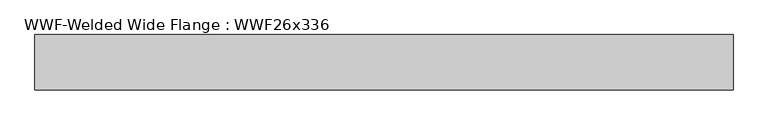
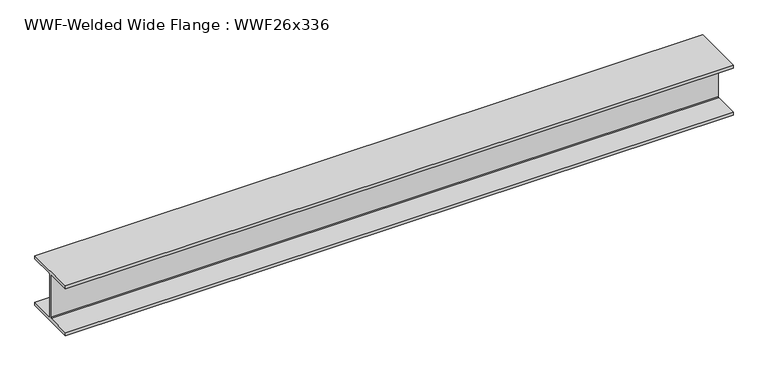
"""IFC4 building model written with IfcOpenShell, lengths in millimetres: beam geometry, WWF-Welded Wide Flange : WWF26x336."""

from ifc_helpers import new_model, si_unit, frame, origin, place, context, project, spatial, polyline, outline, extrude, source, transform, mapped, element, save


def wwf_welded_wide_flange_wwf26x336_e7b07e13(model_context):
    return source(origin(), model_context, "Body", "SweptSolid", [
        extrude(outline(polyline([(324.993, -284.988), (324.993, -324.993), (-324.993, -324.993), (-324.993, -284.988), (-20.6375, -284.988), (-9.9949, -274.3454), (-9.9949, 274.3454), (-20.6375, 284.988), (-324.993, 284.988), (-324.993, 324.993), (324.993, 324.993), (324.993, 284.988), (20.6375, 284.988), (9.9949, 274.3454), (9.9949, -274.3454), (20.6375, -284.988), (324.993, -284.988)])), frame((-4157.4839163, 0.0, 0.0), z_axis=(1.0, 0.0, 0.0), x_axis=(0.0, 1.0, 0.0)), (0.0, 0.0, 1.0), 8221.7226263),
    ])


if __name__ == "__main__":
    model = new_model("IFC4")
    model_context = context("Model", 3, world=origin())
    ifc_project = project(units=[si_unit("LENGTHUNIT", "METRE", prefix="MILLI")], contexts=[model_context])
    site = spatial("IfcSite", under=ifc_project)
    building = spatial("IfcBuilding", under=site)
    placement = place(None, origin())
    wwf_welded_wide_flange_wwf26x336_shape = wwf_welded_wide_flange_wwf26x336_e7b07e13(model_context)
    element("IfcBeam", 1, ObjectType="WWF-Welded Wide Flange : WWF26x336", at=placement, inside=building, context=model_context, shape_type="MappedRepresentation", body=[
        mapped(wwf_welded_wide_flange_wwf26x336_shape, transform((0.0, 0.0, 0.0), x_axis=(1.0, 0.0, 0.0), y_axis=(0.0, 1.0, 0.0), z_axis=(0.0, 0.0, 1.0))),
    ])
    save(model, "model.ifc")

# Revit data of these elements
# Type "WWF-Welded Wide Flange : WWF26x336"
#   Assembly Code = "B10"
#   Nominal d = "12"
#   W = 336
#   Length [instance default] = 1524 mm
#   bf = 649.986 mm
#   d = 649.986 mm
#   k = 20.638 mm
#   tf = 40.005 mm
#   tw = 19.99 mm
#   A = 0.0635483 m²
#   Structural Material [instance default] = Steel ASTM A572
# Element 1 (IfcBeam, "WWF-Welded Wide Flange : WWF26x336")
#   Structural Material = Metal - Steel 43-275
#   Materials on its faces: "Metal - Steel 43-275"
# Materials
#   "Steel ASTM A572": class "Metal", colour RGB 247 247 247, transparency 0, Description = "Structural steel, high strength low alloy, ASTM - A572 - 50", Cost = 0
#   "Metal - Steel 43-275": class "Metal", colour RGB 247 247 247, transparency 0, Cost = 0
